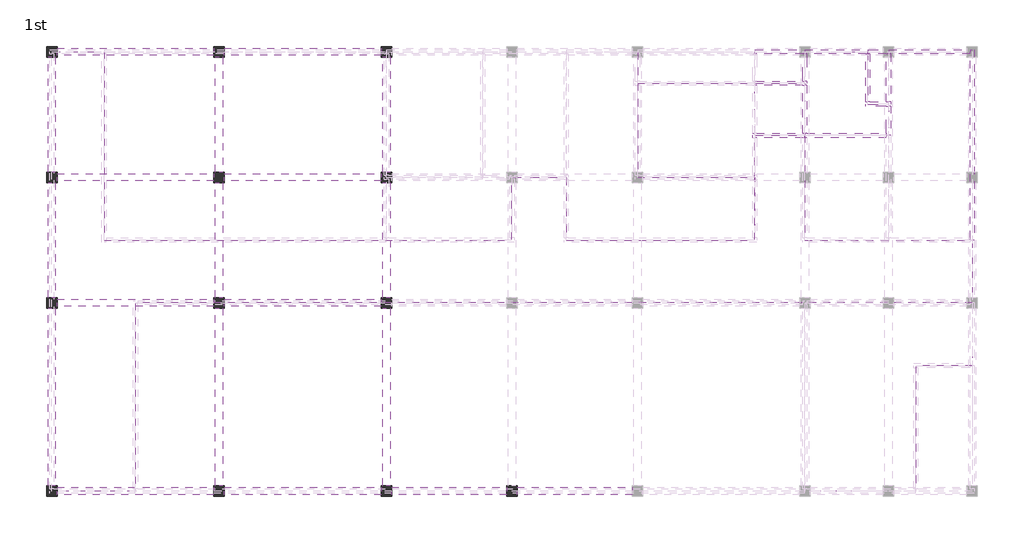
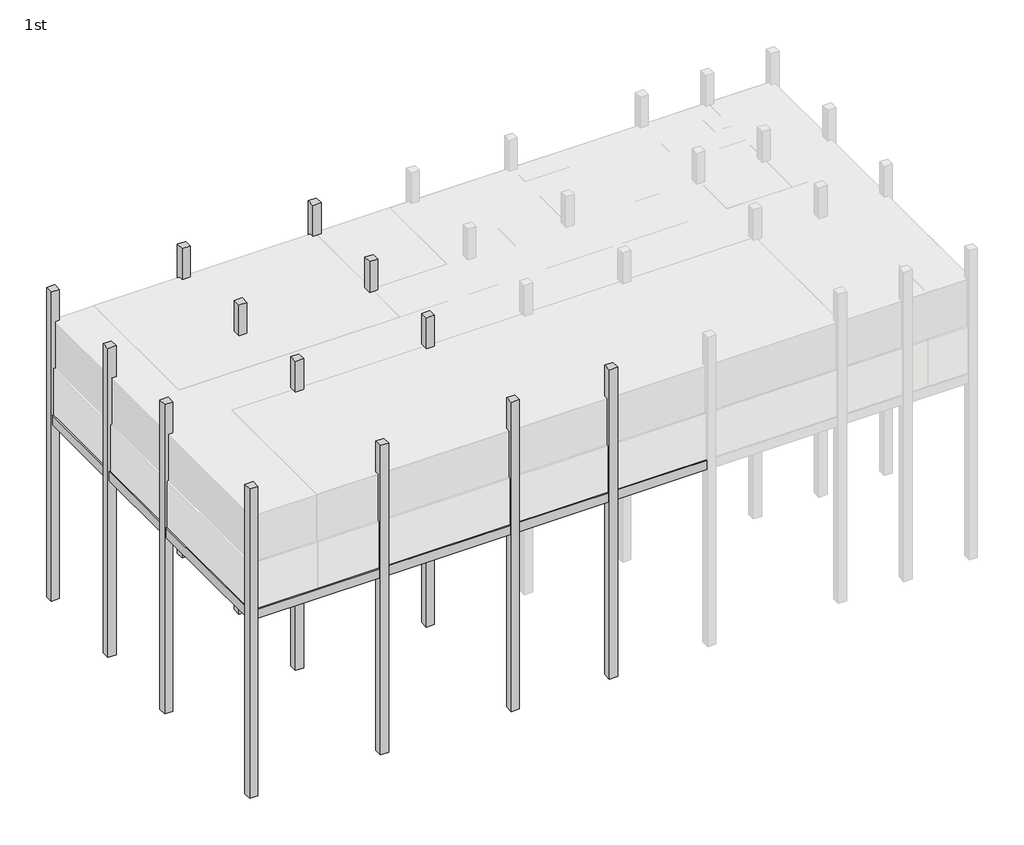
# One storey, part 2 of 3: 19 beams, 17 slabs, 14 walls, 13 columns.
"""IFC4 building model written with IfcOpenShell, lengths in millimetres."""

from ifc_helpers import new_model, si_unit, frame, origin, origin_with_axes, place, context, project, spatial, polyline, outline, extrude, faceted_brep, element, save

model = new_model("IFC4")

# Units and contexts
model_context = context("Model", 3, world=origin())
ifc_project = project(units=[si_unit("LENGTHUNIT", "METRE", prefix="MILLI")], contexts=[model_context])

# Site, building, storey
site = spatial("IfcSite", under=ifc_project)
building = spatial("IfcBuilding", under=site)
storey = spatial("IfcBuildingStorey", under=building, Name="1st", Elevation=6000.0)

# Beams
placement = place(None, origin())
element("IfcBeam", 1, ObjectType="Concrete-Rectangular-Beam : BM111_400x500_RG1", at=placement, inside=storey, context=model_context, shape_type="SweptSolid", body=[
    extrude(outline(polyline([(45284.6521483, 184673.8614395), (45634.6521483, 184673.8614395), (45634.6521483, 179173.8614395), (45284.6521483, 179173.8614395), (45284.6521483, 184673.8614395)])), frame((0.0, 0.0, 11400.0), z_axis=(0.0, 0.0, 1.0), x_axis=(1.0, 0.0, 0.0)), (0.0, 0.0, 1.0), 600.0),
])
element("IfcBeam", 2, ObjectType="Concrete-Rectangular-Beam : BM111_400x500_RG1", at=placement, inside=storey, context=model_context, shape_type="SweptSolid", body=[
    extrude(outline(polyline([(45284.6521483, 178673.8614395), (45634.6521483, 178673.8614395), (45634.6521483, 173173.8614395), (45284.6521483, 173173.8614395), (45284.6521483, 178673.8614395)])), frame((0.0, 0.0, 11400.0), z_axis=(0.0, 0.0, 1.0), x_axis=(1.0, 0.0, 0.0)), (0.0, 0.0, 1.0), 600.0),
])
element("IfcBeam", 3, ObjectType="Concrete-Rectangular-Beam : BM111_400x500_RG1", at=placement, inside=storey, context=model_context, shape_type="SweptSolid", body=[
    extrude(outline(polyline([(45284.6521483, 172673.8614395), (45634.6521483, 172673.8614395), (45634.6521483, 164173.8614395), (45284.6521483, 164173.8614395), (45284.6521483, 172673.8614395)])), frame((0.0, 0.0, 11400.0), z_axis=(0.0, 0.0, 1.0), x_axis=(1.0, 0.0, 0.0)), (0.0, 0.0, 1.0), 600.0),
])
element("IfcBeam", 4, ObjectType="Concrete-Rectangular-Beam : BM111_400x500_RG1", at=placement, inside=storey, context=model_context, shape_type="SweptSolid", body=[
    extrude(outline(polyline([(53284.6521483, 184673.8614395), (53634.6521483, 184673.8614395), (53634.6521483, 179173.8614395), (53284.6521483, 179173.8614395), (53284.6521483, 184673.8614395)])), frame((0.0, 0.0, 11400.0), z_axis=(0.0, 0.0, 1.0), x_axis=(1.0, 0.0, 0.0)), (0.0, 0.0, 1.0), 600.0),
])
element("IfcBeam", 5, ObjectType="Concrete-Rectangular-Beam : BM111_400x500_RG1", at=placement, inside=storey, context=model_context, shape_type="SweptSolid", body=[
    extrude(outline(polyline([(53284.6521483, 178673.8614395), (53634.6521483, 178673.8614395), (53634.6521483, 173173.8614395), (53284.6521483, 173173.8614395), (53284.6521483, 178673.8614395)])), frame((0.0, 0.0, 11400.0), z_axis=(0.0, 0.0, 1.0), x_axis=(1.0, 0.0, 0.0)), (0.0, 0.0, 1.0), 600.0),
])
element("IfcBeam", 6, ObjectType="Concrete-Rectangular-Beam : BM111_400x500_RG1", at=placement, inside=storey, context=model_context, shape_type="SweptSolid", body=[
    extrude(outline(polyline([(53284.6521483, 172673.8614395), (53634.6521483, 172673.8614395), (53634.6521483, 164173.8614395), (53284.6521483, 164173.8614395), (53284.6521483, 172673.8614395)])), frame((0.0, 0.0, 11400.0), z_axis=(0.0, 0.0, 1.0), x_axis=(1.0, 0.0, 0.0)), (0.0, 0.0, 1.0), 600.0),
])
element("IfcBeam", 7, ObjectType="Concrete-Rectangular-Beam : BM111_400x500_RG1", at=placement, inside=storey, context=model_context, shape_type="SweptSolid", body=[
    extrude(outline(polyline([(61284.6521483, 184673.8614395), (61634.6521483, 184673.8614395), (61634.6521483, 179173.8614395), (61284.6521483, 179173.8614395), (61284.6521483, 184673.8614395)])), frame((0.0, 0.0, 11400.0), z_axis=(0.0, 0.0, 1.0), x_axis=(1.0, 0.0, 0.0)), (0.0, 0.0, 1.0), 600.0),
])
element("IfcBeam", 8, ObjectType="Concrete-Rectangular-Beam : BM111_400x500_RG1", at=placement, inside=storey, context=model_context, shape_type="SweptSolid", body=[
    extrude(outline(polyline([(61284.6521483, 178673.8614395), (61634.6521483, 178673.8614395), (61634.6521483, 173173.8614395), (61284.6521483, 173173.8614395), (61284.6521483, 178673.8614395)])), frame((0.0, 0.0, 11400.0), z_axis=(0.0, 0.0, 1.0), x_axis=(1.0, 0.0, 0.0)), (0.0, 0.0, 1.0), 600.0),
])
element("IfcBeam", 9, ObjectType="Concrete-Rectangular-Beam : BM111_400x500_RG1", at=placement, inside=storey, context=model_context, shape_type="SweptSolid", body=[
    extrude(outline(polyline([(61284.6521483, 172673.8614395), (61634.6521483, 172673.8614395), (61634.6521483, 164173.8614395), (61284.6521483, 164173.8614395), (61284.6521483, 172673.8614395)])), frame((0.0, 0.0, 11400.0), z_axis=(0.0, 0.0, 1.0), x_axis=(1.0, 0.0, 0.0)), (0.0, 0.0, 1.0), 600.0),
])
element("IfcBeam", 10, ObjectType="Concrete-Rectangular-Beam : BM111_400x500_RG1", at=placement, inside=storey, context=model_context, shape_type="SweptSolid", body=[
    extrude(outline(polyline([(45709.6521483, 184748.8614395), (45709.6521483, 185098.8614395), (53209.6521483, 185098.8614395), (53209.6521483, 184748.8614395), (45709.6521483, 184748.8614395)])), frame((0.0, 0.0, 11400.0), z_axis=(0.0, 0.0, 1.0), x_axis=(1.0, 0.0, 0.0)), (0.0, 0.0, 1.0), 600.0),
])
element("IfcBeam", 11, ObjectType="Concrete-Rectangular-Beam : BM111_400x500_RG1", at=placement, inside=storey, context=model_context, shape_type="SweptSolid", body=[
    extrude(outline(polyline([(53709.6521483, 184748.8614395), (53709.6521483, 185098.8614395), (61209.6521483, 185098.8614395), (61209.6521483, 184748.8614395), (53709.6521483, 184748.8614395)])), frame((0.0, 0.0, 11400.0), z_axis=(0.0, 0.0, 1.0), x_axis=(1.0, 0.0, 0.0)), (0.0, 0.0, 1.0), 600.0),
])
element("IfcBeam", 12, ObjectType="Concrete-Rectangular-Beam : BM111_400x500_RG1", at=placement, inside=storey, context=model_context, shape_type="SweptSolid", body=[
    extrude(outline(polyline([(45709.6521483, 178748.8614395), (45709.6521483, 179098.8614395), (53209.6521483, 179098.8614395), (53209.6521483, 178748.8614395), (45709.6521483, 178748.8614395)])), frame((0.0, 0.0, 11400.0), z_axis=(0.0, 0.0, 1.0), x_axis=(1.0, 0.0, 0.0)), (0.0, 0.0, 1.0), 600.0),
])
element("IfcBeam", 13, ObjectType="Concrete-Rectangular-Beam : BM111_400x500_RG1", at=placement, inside=storey, context=model_context, shape_type="SweptSolid", body=[
    extrude(outline(polyline([(53709.6521483, 178748.8614395), (53709.6521483, 179098.8614395), (61209.6521483, 179098.8614395), (61209.6521483, 178748.8614395), (53709.6521483, 178748.8614395)])), frame((0.0, 0.0, 11400.0), z_axis=(0.0, 0.0, 1.0), x_axis=(1.0, 0.0, 0.0)), (0.0, 0.0, 1.0), 600.0),
])
element("IfcBeam", 14, ObjectType="Concrete-Rectangular-Beam : BM111_400x500_RG1", at=placement, inside=storey, context=model_context, shape_type="SweptSolid", body=[
    extrude(outline(polyline([(45709.6521483, 172748.8614395), (45709.6521483, 173098.8614395), (53209.6521483, 173098.8614395), (53209.6521483, 172748.8614395), (45709.6521483, 172748.8614395)])), frame((0.0, 0.0, 11400.0), z_axis=(0.0, 0.0, 1.0), x_axis=(1.0, 0.0, 0.0)), (0.0, 0.0, 1.0), 600.0),
])
element("IfcBeam", 15, ObjectType="Concrete-Rectangular-Beam : BM111_400x500_RG1", at=placement, inside=storey, context=model_context, shape_type="SweptSolid", body=[
    extrude(outline(polyline([(53709.6521483, 172748.8614395), (53709.6521483, 173098.8614395), (61209.6521483, 173098.8614395), (61209.6521483, 172748.8614395), (53709.6521483, 172748.8614395)])), frame((0.0, 0.0, 11400.0), z_axis=(0.0, 0.0, 1.0), x_axis=(1.0, 0.0, 0.0)), (0.0, 0.0, 1.0), 600.0),
])
element("IfcBeam", 16, ObjectType="Concrete-Rectangular-Beam : BM111_400x500_RG1", at=placement, inside=storey, context=model_context, shape_type="SweptSolid", body=[
    extrude(outline(polyline([(45709.6521483, 163748.8614395), (45709.6521483, 164098.8614395), (53209.6521483, 164098.8614395), (53209.6521483, 163748.8614395), (45709.6521483, 163748.8614395)])), frame((0.0, 0.0, 11400.0), z_axis=(0.0, 0.0, 1.0), x_axis=(1.0, 0.0, 0.0)), (0.0, 0.0, 1.0), 600.0),
])
element("IfcBeam", 17, ObjectType="Concrete-Rectangular-Beam : BM111_400x500_RG1", at=placement, inside=storey, context=model_context, shape_type="SweptSolid", body=[
    extrude(outline(polyline([(53709.6521483, 163748.8614395), (53709.6521483, 164098.8614395), (61209.6521483, 164098.8614395), (61209.6521483, 163748.8614395), (53709.6521483, 163748.8614395)])), frame((0.0, 0.0, 11400.0), z_axis=(0.0, 0.0, 1.0), x_axis=(1.0, 0.0, 0.0)), (0.0, 0.0, 1.0), 600.0),
])
element("IfcBeam", 18, ObjectType="Concrete-Rectangular-Beam : BM111_400x500_RG1", at=placement, inside=storey, context=model_context, shape_type="SweptSolid", body=[
    extrude(outline(polyline([(61709.6521483, 163748.8614395), (61709.6521483, 164098.8614395), (67209.6521483, 164098.8614395), (67209.6521483, 163748.8614395), (61709.6521483, 163748.8614395)])), frame((0.0, 0.0, 11400.0), z_axis=(0.0, 0.0, 1.0), x_axis=(1.0, 0.0, 0.0)), (0.0, 0.0, 1.0), 600.0),
])
element("IfcBeam", 19, ObjectType="Concrete-Rectangular-Beam : BM111_400x500_RG1", at=placement, inside=storey, context=model_context, shape_type="SweptSolid", body=[
    extrude(outline(polyline([(67709.6521483, 163748.8614395), (67709.6521483, 164098.8614395), (73209.6521483, 164098.8614395), (73209.6521483, 163748.8614395), (67709.6521483, 163748.8614395)])), frame((0.0, 0.0, 11400.0), z_axis=(0.0, 0.0, 1.0), x_axis=(1.0, 0.0, 0.0)), (0.0, 0.0, 1.0), 600.0),
])

# Columns
element("IfcColumn", 20, ObjectType="Concrete-Rectangular-Column : CL111_500x500", at=placement, inside=storey, context=model_context, shape_type="SweptSolid", body=[
    extrude(outline(polyline([(45709.6521483, 185173.8614395), (45709.6521483, 184673.8614395), (45209.6521483, 184673.8614395), (45209.6521483, 185173.8614395), (45709.6521483, 185173.8614395)])), origin_with_axes(), (0.0, 0.0, 1.0), 20000.0),
])
element("IfcColumn", 21, ObjectType="Concrete-Rectangular-Column : CL111_500x500", at=placement, inside=storey, context=model_context, shape_type="SweptSolid", body=[
    extrude(outline(polyline([(45709.6521483, 179173.8614395), (45709.6521483, 178673.8614395), (45209.6521483, 178673.8614395), (45209.6521483, 179173.8614395), (45709.6521483, 179173.8614395)])), origin_with_axes(), (0.0, 0.0, 1.0), 20000.0),
])
element("IfcColumn", 22, ObjectType="Concrete-Rectangular-Column : CL111_500x500", at=placement, inside=storey, context=model_context, shape_type="SweptSolid", body=[
    extrude(outline(polyline([(45709.6521483, 173173.8614395), (45709.6521483, 172673.8614395), (45209.6521483, 172673.8614395), (45209.6521483, 173173.8614395), (45709.6521483, 173173.8614395)])), origin_with_axes(), (0.0, 0.0, 1.0), 20000.0),
])
element("IfcColumn", 23, ObjectType="Concrete-Rectangular-Column : CL111_500x500", at=placement, inside=storey, context=model_context, shape_type="SweptSolid", body=[
    extrude(outline(polyline([(45709.6521483, 164173.8614395), (45709.6521483, 163673.8614395), (45209.6521483, 163673.8614395), (45209.6521483, 164173.8614395), (45709.6521483, 164173.8614395)])), origin_with_axes(), (0.0, 0.0, 1.0), 20000.0),
])
element("IfcColumn", 24, ObjectType="Concrete-Rectangular-Column : CL111_500x500", at=placement, inside=storey, context=model_context, shape_type="SweptSolid", body=[
    extrude(outline(polyline([(53709.6521483, 185173.8614395), (53709.6521483, 184673.8614395), (53209.6521483, 184673.8614395), (53209.6521483, 185173.8614395), (53709.6521483, 185173.8614395)])), origin_with_axes(), (0.0, 0.0, 1.0), 20000.0),
])
element("IfcColumn", 25, ObjectType="Concrete-Rectangular-Column : CL111_500x500", at=placement, inside=storey, context=model_context, shape_type="SweptSolid", body=[
    extrude(outline(polyline([(53709.6521483, 179173.8614395), (53709.6521483, 178673.8614395), (53209.6521483, 178673.8614395), (53209.6521483, 179173.8614395), (53709.6521483, 179173.8614395)])), origin_with_axes(), (0.0, 0.0, 1.0), 20000.0),
])
element("IfcColumn", 26, ObjectType="Concrete-Rectangular-Column : CL111_500x500", at=placement, inside=storey, context=model_context, shape_type="SweptSolid", body=[
    extrude(outline(polyline([(53709.6521483, 173173.8614395), (53709.6521483, 172673.8614395), (53209.6521483, 172673.8614395), (53209.6521483, 173173.8614395), (53709.6521483, 173173.8614395)])), origin_with_axes(), (0.0, 0.0, 1.0), 20000.0),
])
element("IfcColumn", 27, ObjectType="Concrete-Rectangular-Column : CL111_500x500", at=placement, inside=storey, context=model_context, shape_type="SweptSolid", body=[
    extrude(outline(polyline([(53709.6521483, 164173.8614395), (53709.6521483, 163673.8614395), (53209.6521483, 163673.8614395), (53209.6521483, 164173.8614395), (53709.6521483, 164173.8614395)])), origin_with_axes(), (0.0, 0.0, 1.0), 20000.0),
])
element("IfcColumn", 28, ObjectType="Concrete-Rectangular-Column : CL111_500x500", at=placement, inside=storey, context=model_context, shape_type="SweptSolid", body=[
    extrude(outline(polyline([(61709.6521483, 185173.8614395), (61709.6521483, 184673.8614395), (61209.6521483, 184673.8614395), (61209.6521483, 185173.8614395), (61709.6521483, 185173.8614395)])), origin_with_axes(), (0.0, 0.0, 1.0), 20000.0),
])
element("IfcColumn", 29, ObjectType="Concrete-Rectangular-Column : CL111_500x500", at=placement, inside=storey, context=model_context, shape_type="SweptSolid", body=[
    extrude(outline(polyline([(61709.6521483, 179173.8614395), (61709.6521483, 178673.8614395), (61209.6521483, 178673.8614395), (61209.6521483, 179173.8614395), (61709.6521483, 179173.8614395)])), origin_with_axes(), (0.0, 0.0, 1.0), 20000.0),
])
element("IfcColumn", 30, ObjectType="Concrete-Rectangular-Column : CL111_500x500", at=placement, inside=storey, context=model_context, shape_type="SweptSolid", body=[
    extrude(outline(polyline([(61709.6521483, 173173.8614395), (61709.6521483, 172673.8614395), (61209.6521483, 172673.8614395), (61209.6521483, 173173.8614395), (61709.6521483, 173173.8614395)])), origin_with_axes(), (0.0, 0.0, 1.0), 20000.0),
])
element("IfcColumn", 31, ObjectType="Concrete-Rectangular-Column : CL111_500x500", at=placement, inside=storey, context=model_context, shape_type="SweptSolid", body=[
    extrude(outline(polyline([(61709.6521483, 164173.8614395), (61709.6521483, 163673.8614395), (61209.6521483, 163673.8614395), (61209.6521483, 164173.8614395), (61709.6521483, 164173.8614395)])), origin_with_axes(), (0.0, 0.0, 1.0), 20000.0),
])
element("IfcColumn", 32, ObjectType="Concrete-Rectangular-Column : CL111_500x500", at=placement, inside=storey, context=model_context, shape_type="SweptSolid", body=[
    extrude(outline(polyline([(67709.6521483, 164173.8614395), (67709.6521483, 163673.8614395), (67209.6521483, 163673.8614395), (67209.6521483, 164173.8614395), (67709.6521483, 164173.8614395)])), origin_with_axes(), (0.0, 0.0, 1.0), 20000.0),
])

# Slabs
element("IfcSlab", 33, ObjectType="CFS11_Slab RC_T150", at=placement, inside=storey, context=model_context, shape_type="SweptSolid", body=[
    extrude(outline(polyline([(49459.6521483, 172923.8614395), (81459.6521483, 172923.8614395), (81459.6521483, 163923.8614395), (49459.6521483, 163923.8614395), (49459.6521483, 172923.8614395)])), frame((0.0, 0.0, 11850.0), z_axis=(0.0, 0.0, 1.0), x_axis=(1.0, 0.0, 0.0)), (0.0, 0.0, 1.0), 150.0),
])
element("IfcSlab", 34, ObjectType="CFS11_Slab RC_T150", at=placement, inside=storey, context=model_context, shape_type="SweptSolid", body=[
    extrude(outline(polyline([(47959.6521483, 184923.8614395), (61459.6521483, 184923.8614395), (61459.6521483, 175923.8614395), (47959.6521483, 175923.8614395), (47959.6521483, 184923.8614395)])), frame((0.0, 0.0, 11850.0), z_axis=(0.0, 0.0, 1.0), x_axis=(1.0, 0.0, 0.0)), (0.0, 0.0, 1.0), 150.0),
])
element("IfcSlab", 35, ObjectType="CFS11_Slab RC_T150", at=placement, inside=storey, context=model_context, shape_type="SweptSolid", body=[
    extrude(outline(polyline([(61459.6521483, 178923.8614395), (61459.6521483, 184923.8614395), (66059.6521483, 184923.8614395), (66059.6521483, 178923.8614395), (61459.6521483, 178923.8614395)])), frame((0.0, 0.0, 11850.0), z_axis=(0.0, 0.0, 1.0), x_axis=(1.0, 0.0, 0.0)), (0.0, 0.0, 1.0), 150.0),
])
element("IfcSlab", 36, ObjectType="CFS11_Slab RC_T150", at=placement, inside=storey, context=model_context, shape_type="SweptSolid", body=[
    extrude(outline(polyline([(81459.6521483, 175923.8614395), (81459.6521483, 180923.8614395), (85459.6521483, 180923.8614395), (85459.6521483, 175923.8614395), (81459.6521483, 175923.8614395)])), frame((0.0, 0.0, 11850.0), z_axis=(0.0, 0.0, 1.0), x_axis=(1.0, 0.0, 0.0)), (0.0, 0.0, 1.0), 150.0),
])
element("IfcSlab", 37, ObjectType="CFS11_Slab RC_T150", at=placement, inside=storey, context=model_context, shape_type="SweptSolid", body=[
    extrude(outline(polyline([(89459.6521483, 175923.8614395), (85459.6521483, 175923.8614395), (85459.6521483, 184923.8614395), (89459.6521483, 184923.8614395), (89459.6521483, 175923.8614395)])), frame((0.0, 0.0, 11850.0), z_axis=(0.0, 0.0, 1.0), x_axis=(1.0, 0.0, 0.0)), (0.0, 0.0, 1.0), 150.0),
])
element("IfcSlab", 38, ObjectType="CFS11_Slab RC_T150", at=placement, inside=storey, context=model_context, shape_type="SweptSolid", body=[
    extrude(outline(polyline([(66059.6521483, 178923.8614395), (66059.6521483, 184923.8614395), (70059.6521483, 184923.8614395), (70059.6521483, 178923.8614395), (66059.6521483, 178923.8614395)])), frame((0.0, 0.0, 11850.0), z_axis=(0.0, 0.0, 1.0), x_axis=(1.0, 0.0, 0.0)), (0.0, 0.0, 1.0), 150.0),
])
element("IfcSlab", 39, ObjectType="CFS11_Slab RC_T150", at=placement, inside=storey, context=model_context, shape_type="SweptSolid", body=[
    extrude(outline(polyline([(61459.6521483, 175923.8614395), (61459.6521483, 178923.8614395), (67459.6521483, 178923.8614395), (67459.6521483, 175923.8614395), (61459.6521483, 175923.8614395)])), frame((0.0, 0.0, 11850.0), z_axis=(0.0, 0.0, 1.0), x_axis=(1.0, 0.0, 0.0)), (0.0, 0.0, 1.0), 150.0),
])
element("IfcSlab", 40, ObjectType="CFS11_Slab RC_T150", at=placement, inside=storey, context=model_context, shape_type="SweptSolid", body=[
    extrude(outline(polyline([(79059.6521483, 183423.8614395), (79059.6521483, 184923.8614395), (81459.6521483, 184923.8614395), (81459.6521483, 183423.8614395), (79059.6521483, 183423.8614395)])), frame((0.0, 0.0, 11850.0), z_axis=(0.0, 0.0, 1.0), x_axis=(1.0, 0.0, 0.0)), (0.0, 0.0, 1.0), 150.0),
])
element("IfcSlab", 41, ObjectType="CFS11_Slab RC_T150", at=placement, inside=storey, context=model_context, shape_type="SweptSolid", body=[
    extrude(outline(polyline([(89459.6521483, 172923.8614395), (49459.6521483, 172923.8614395), (49459.6521483, 163923.8614395), (45459.6521483, 163923.8614395), (45459.6521483, 184923.8614395), (47959.6521483, 184923.8614395), (47959.6521483, 175923.8614395), (67459.6521483, 175923.8614395), (67459.6521483, 178923.8614395), (70059.6521483, 178923.8614395), (70059.6521483, 175923.8614395), (79059.6521483, 175923.8614395), (79059.6521483, 180923.8614395), (81459.6521483, 180923.8614395), (81459.6521483, 175923.8614395), (89459.6521483, 175923.8614395), (89459.6521483, 172923.8614395)])), frame((0.0, 0.0, 11850.0), z_axis=(0.0, 0.0, 1.0), x_axis=(1.0, 0.0, 0.0)), (0.0, 0.0, 1.0), 150.0),
])
element("IfcSlab", 42, ObjectType="CFS11_Slab RC_T150", at=placement, inside=storey, context=model_context, shape_type="SweptSolid", body=[
    extrude(outline(polyline([(79059.6521483, 180923.8614395), (79059.6521483, 183423.8614395), (81459.6521483, 183423.8614395), (81459.6521483, 180923.8614395), (79059.6521483, 180923.8614395)])), frame((0.0, 0.0, 11850.0), z_axis=(0.0, 0.0, 1.0), x_axis=(1.0, 0.0, 0.0)), (0.0, 0.0, 1.0), 150.0),
])
element("IfcSlab", 43, ObjectType="CFS11_Slab RC_T150", at=placement, inside=storey, context=model_context, shape_type="SweptSolid", body=[
    extrude(outline(polyline([(73459.6521483, 184923.8614395), (79059.6521483, 184923.8614395), (79059.6521483, 183423.8614395), (73459.6521483, 183423.8614395), (73459.6521483, 184923.8614395)])), frame((0.0, 0.0, 11850.0), z_axis=(0.0, 0.0, 1.0), x_axis=(1.0, 0.0, 0.0)), (0.0, 0.0, 1.0), 150.0),
])
element("IfcSlab", 44, ObjectType="CFS11_Slab RC_T150", at=placement, inside=storey, context=model_context, shape_type="SweptSolid", body=[
    extrude(outline(polyline([(79059.6521483, 175923.8614395), (70059.6521483, 175923.8614395), (70059.6521483, 184923.8614395), (73459.6521483, 184923.8614395), (73459.6521483, 178923.8614395), (79059.6521483, 178923.8614395), (79059.6521483, 175923.8614395)])), frame((0.0, 0.0, 11850.0), z_axis=(0.0, 0.0, 1.0), x_axis=(1.0, 0.0, 0.0)), (0.0, 0.0, 1.0), 150.0),
])
element("IfcSlab", 45, ObjectType="CFS11_Slab RC_T150", at=placement, inside=storey, context=model_context, shape_type="SweptSolid", body=[
    extrude(outline(polyline([(73459.6521483, 183423.8614395), (79059.6521483, 183423.8614395), (79059.6521483, 178923.8614395), (73459.6521483, 178923.8614395), (73459.6521483, 183423.8614395)])), frame((0.0, 0.0, 11850.0), z_axis=(0.0, 0.0, 1.0), x_axis=(1.0, 0.0, 0.0)), (0.0, 0.0, 1.0), 150.0),
])
element("IfcSlab", 46, ObjectType="CFS11_Slab RC_T150", at=placement, inside=storey, context=model_context, shape_type="SweptSolid", body=[
    extrude(outline(polyline([(81459.6521483, 163923.8614395), (81459.6521483, 172923.8614395), (89459.6521483, 172923.8614395), (89459.6521483, 169923.8614395), (86759.6521483, 169923.8614395), (86759.6521483, 163923.8614395), (81459.6521483, 163923.8614395)])), frame((0.0, 0.0, 11850.0), z_axis=(0.0, 0.0, 1.0), x_axis=(1.0, 0.0, 0.0)), (0.0, 0.0, 1.0), 150.0),
])
element("IfcSlab", 47, ObjectType="CFS11_Slab RC_T150", at=placement, inside=storey, context=model_context, shape_type="SweptSolid", body=[
    extrude(outline(polyline([(89459.6521483, 169923.8614395), (89459.6521483, 163923.8614395), (86759.6521483, 163923.8614395), (86759.6521483, 169923.8614395), (89459.6521483, 169923.8614395)])), frame((0.0, 0.0, 11850.0), z_axis=(0.0, 0.0, 1.0), x_axis=(1.0, 0.0, 0.0)), (0.0, 0.0, 1.0), 150.0),
])
element("IfcSlab", 48, ObjectType="CFS11_Slab RC_T150", at=placement, inside=storey, context=model_context, shape_type="SweptSolid", body=[
    extrude(outline(polyline([(85459.6521483, 180923.8614395), (81459.6521483, 180923.8614395), (81459.6521483, 184923.8614395), (84459.6521483, 184923.8614395), (84459.6521483, 182423.8614395), (85459.6521483, 182423.8614395), (85459.6521483, 180923.8614395)])), frame((0.0, 0.0, 11850.0), z_axis=(0.0, 0.0, 1.0), x_axis=(1.0, 0.0, 0.0)), (0.0, 0.0, 1.0), 150.0),
])
element("IfcSlab", 49, ObjectType="CFS11_Slab RC_T150", at=placement, inside=storey, context=model_context, shape_type="SweptSolid", body=[
    extrude(outline(polyline([(84459.6521483, 184923.8614395), (85459.6521483, 184923.8614395), (85459.6521483, 182423.8614395), (84459.6521483, 182423.8614395), (84459.6521483, 184923.8614395)])), frame((0.0, 0.0, 11850.0), z_axis=(0.0, 0.0, 1.0), x_axis=(1.0, 0.0, 0.0)), (0.0, 0.0, 1.0), 150.0),
])

# Walls
element("IfcWall", 50, ObjectType="WA111-Exterior RC Wall 200mm", at=placement, inside=storey, context=model_context, shape_type="Brep", body=[
    faceted_brep([(89559.6521483, 175923.8614395, 12000.0), (89559.6521483, 185023.8614395, 12000.0), (89559.6521483, 185023.8614395, 15000.0), (89559.6521483, 175923.8614395, 15000.0), (89359.6521483, 175923.8614395, 12000.0), (89359.6521483, 175923.8614395, 15000.0), (89359.6521483, 176023.8614395, 15000.0), (89359.6521483, 184823.8614395, 15000.0), (89359.6521483, 185023.8614395, 15000.0), (89359.6521483, 185023.8614395, 12000.0), (89359.6521483, 184823.8614395, 12000.0), (89359.6521483, 176023.8614395, 12000.0)], [[[0, 1, 2, 3]], [[4, 5, 6, 7, 8, 9, 10, 11]], [[1, 0, 4, 11, 10, 9]], [[3, 2, 8, 7, 6, 5]], [[0, 3, 5, 4]], [[2, 1, 9, 8]]]),
])
element("IfcWall", 51, ObjectType="WA111-Exterior RC Wall 200mm", at=placement, inside=storey, context=model_context, shape_type="Brep", body=[
    faceted_brep([(89359.6521483, 185023.8614395, 12000.0), (85459.6521483, 185023.8614395, 12000.0), (85459.6521483, 185023.8614395, 15000.0), (89359.6521483, 185023.8614395, 15000.0), (89359.6521483, 184823.8614395, 12000.0), (89359.6521483, 184823.8614395, 15000.0), (85559.6521483, 184823.8614395, 15000.0), (85459.6521483, 184823.8614395, 15000.0), (85459.6521483, 184823.8614395, 12000.0), (85559.6521483, 184823.8614395, 12000.0)], [[[0, 1, 2, 3]], [[4, 5, 6, 7, 8, 9]], [[1, 0, 4, 9, 8]], [[2, 1, 8, 7]], [[3, 2, 7, 6, 5]], [[0, 3, 5, 4]]]),
])
element("IfcWall", 52, ObjectType="WA111-Exterior RC Wall 200mm", at=placement, inside=storey, context=model_context, shape_type="Brep", body=[
    faceted_brep([(81459.6521483, 185023.8614395, 12000.0), (79059.6521483, 185023.8614395, 12000.0), (79059.6521483, 185023.8614395, 15000.0), (81459.6521483, 185023.8614395, 15000.0), (81459.6521483, 184823.8614395, 12000.0), (81459.6521483, 184823.8614395, 15000.0), (81359.6521483, 184823.8614395, 15000.0), (79159.6521483, 184823.8614395, 15000.0), (79059.6521483, 184823.8614395, 15000.0), (79059.6521483, 184823.8614395, 12000.0), (79159.6521483, 184823.8614395, 12000.0), (81359.6521483, 184823.8614395, 12000.0)], [[[0, 1, 2, 3]], [[4, 5, 6, 7, 8, 9, 10, 11]], [[1, 0, 4, 11, 10, 9]], [[2, 1, 9, 8]], [[3, 2, 8, 7, 6, 5]], [[0, 3, 5, 4]]]),
])
element("IfcWall", 53, ObjectType="WA111-Exterior RC Wall 200mm", at=placement, inside=storey, context=model_context, shape_type="Brep", body=[
    faceted_brep([(84459.6521483, 185023.8614395, 12000.0), (81459.6521483, 185023.8614395, 12000.0), (81459.6521483, 185023.8614395, 15000.0), (84459.6521483, 185023.8614395, 15000.0), (84459.6521483, 184823.8614395, 12000.0), (84459.6521483, 184823.8614395, 15000.0), (84359.6521483, 184823.8614395, 15000.0), (81559.6521483, 184823.8614395, 15000.0), (81459.6521483, 184823.8614395, 15000.0), (81459.6521483, 184823.8614395, 12000.0), (81559.6521483, 184823.8614395, 12000.0), (84359.6521483, 184823.8614395, 12000.0)], [[[0, 1, 2, 3]], [[4, 5, 6, 7, 8, 9, 10, 11]], [[1, 0, 4, 11, 10, 9]], [[2, 1, 9, 8]], [[3, 2, 8, 7, 6, 5]], [[0, 3, 5, 4]]]),
])
element("IfcWall", 54, ObjectType="WA111-Exterior RC Wall 200mm", at=placement, inside=storey, context=model_context, shape_type="Brep", body=[
    faceted_brep([(85459.6521483, 185023.8614395, 12000.0), (84459.6521483, 185023.8614395, 12000.0), (84459.6521483, 185023.8614395, 15000.0), (85459.6521483, 185023.8614395, 15000.0), (85459.6521483, 184823.8614395, 12000.0), (85459.6521483, 184823.8614395, 15000.0), (85359.6521483, 184823.8614395, 15000.0), (84559.6521483, 184823.8614395, 15000.0), (84459.6521483, 184823.8614395, 15000.0), (84459.6521483, 184823.8614395, 12000.0), (84559.6521483, 184823.8614395, 12000.0), (85359.6521483, 184823.8614395, 12000.0)], [[[0, 1, 2, 3]], [[4, 5, 6, 7, 8, 9, 10, 11]], [[1, 0, 4, 11, 10, 9]], [[2, 1, 9, 8]], [[3, 2, 8, 7, 6, 5]], [[0, 3, 5, 4]]]),
])
element("IfcWall", 55, ObjectType="WA121-Interior RC Wall 200mm", at=placement, inside=storey, context=model_context, shape_type="Brep", body=[
    faceted_brep([(85359.6521483, 181023.8614395, 12000.0), (81559.6521483, 181023.8614395, 12000.0), (81459.6521483, 181023.8614395, 12000.0), (81459.6521483, 181023.8614395, 15000.0), (81559.6521483, 181023.8614395, 15000.0), (85359.6521483, 181023.8614395, 15000.0), (85359.6521483, 180823.8614395, 12000.0), (85359.6521483, 180823.8614395, 15000.0), (81559.6521483, 180823.8614395, 15000.0), (81459.6521483, 180823.8614395, 15000.0), (81459.6521483, 180823.8614395, 12000.0), (81559.6521483, 180823.8614395, 12000.0), (85359.6521483, 180923.8614395, 12000.0), (85359.6521483, 180923.8614395, 15000.0)], [[[0, 1, 2, 3, 4, 5]], [[6, 7, 8, 9, 10, 11]], [[2, 1, 0, 12, 6, 11, 10]], [[3, 2, 10, 9]], [[5, 4, 3, 9, 8, 7, 13]], [[0, 5, 13, 7, 6, 12]]]),
])
element("IfcWall", 56, ObjectType="WA121-Interior RC Wall 200mm", at=placement, inside=storey, context=model_context, shape_type="Brep", body=[
    faceted_brep([(85359.6521483, 184823.8614395, 12000.0), (85359.6521483, 182523.8614395, 12000.0), (85359.6521483, 182523.8614395, 15000.0), (85359.6521483, 184823.8614395, 15000.0), (85559.6521483, 184823.8614395, 12000.0), (85559.6521483, 184823.8614395, 15000.0), (85559.6521483, 182523.8614395, 15000.0), (85559.6521483, 182523.8614395, 12000.0), (85459.6521483, 184823.8614395, 12000.0), (85459.6521483, 184823.8614395, 15000.0)], [[[0, 1, 2, 3]], [[4, 5, 6, 7]], [[1, 0, 8, 4, 7]], [[3, 2, 6, 5, 9]], [[0, 3, 9, 5, 4, 8]], [[2, 1, 7, 6]]]),
])
element("IfcWall", 57, ObjectType="WA121-Interior RC Wall 200mm", at=placement, inside=storey, context=model_context, shape_type="Brep", body=[
    faceted_brep([(85359.6521483, 182323.8614395, 12000.0), (85359.6521483, 181023.8614395, 12000.0), (85359.6521483, 180923.8614395, 12000.0), (85359.6521483, 180923.8614395, 15000.0), (85359.6521483, 181023.8614395, 15000.0), (85359.6521483, 182323.8614395, 15000.0), (85559.6521483, 182323.8614395, 12000.0), (85559.6521483, 182323.8614395, 15000.0), (85559.6521483, 180923.8614395, 15000.0), (85559.6521483, 180923.8614395, 12000.0)], [[[0, 1, 2, 3, 4, 5]], [[6, 7, 8, 9]], [[2, 1, 0, 6, 9]], [[3, 2, 9, 8]], [[5, 4, 3, 8, 7]], [[0, 5, 7, 6]]]),
])
element("IfcWall", 58, ObjectType="WA121-Interior RC Wall 200mm", at=placement, inside=storey, context=model_context, shape_type="Brep", body=[
    faceted_brep([(79059.6521483, 183323.8614395, 12000.0), (79159.6521483, 183323.8614395, 12000.0), (81359.6521483, 183323.8614395, 12000.0), (81559.6521483, 183323.8614395, 12000.0), (81559.6521483, 183323.8614395, 15000.0), (81359.6521483, 183323.8614395, 15000.0), (79159.6521483, 183323.8614395, 15000.0), (79059.6521483, 183323.8614395, 15000.0), (79059.6521483, 183523.8614395, 12000.0), (79059.6521483, 183523.8614395, 15000.0), (79159.6521483, 183523.8614395, 15000.0), (81359.6521483, 183523.8614395, 15000.0), (81559.6521483, 183523.8614395, 15000.0), (81559.6521483, 183523.8614395, 12000.0), (81359.6521483, 183523.8614395, 12000.0), (79159.6521483, 183523.8614395, 12000.0)], [[[0, 1, 2, 3, 4, 5, 6, 7]], [[8, 9, 10, 11, 12, 13, 14, 15]], [[3, 2, 1, 0, 8, 15, 14, 13]], [[7, 6, 5, 4, 12, 11, 10, 9]], [[0, 7, 9, 8]], [[4, 3, 13, 12]]]),
])
element("IfcWall", 59, ObjectType="WA121-Interior RC Wall 200mm", at=placement, inside=storey, context=model_context, shape_type="Brep", body=[
    faceted_brep([(81559.6521483, 183523.8614395, 12000.0), (81559.6521483, 184823.8614395, 12000.0), (81559.6521483, 184823.8614395, 15000.0), (81559.6521483, 183523.8614395, 15000.0), (81359.6521483, 183523.8614395, 12000.0), (81359.6521483, 183523.8614395, 15000.0), (81359.6521483, 184823.8614395, 15000.0), (81359.6521483, 184823.8614395, 12000.0), (81459.6521483, 184823.8614395, 12000.0), (81459.6521483, 184823.8614395, 15000.0)], [[[0, 1, 2, 3]], [[4, 5, 6, 7]], [[1, 0, 4, 7, 8]], [[3, 2, 9, 6, 5]], [[2, 1, 8, 7, 6, 9]], [[0, 3, 5, 4]]]),
])
element("IfcWall", 60, ObjectType="WA121-Interior RC Wall 200mm", at=placement, inside=storey, context=model_context, shape_type="Brep", body=[
    faceted_brep([(81459.6521483, 181023.8614395, 12000.0), (81359.6521483, 181023.8614395, 12000.0), (79159.6521483, 181023.8614395, 12000.0), (78959.6521483, 181023.8614395, 12000.0), (78959.6521483, 181023.8614395, 15000.0), (79159.6521483, 181023.8614395, 15000.0), (81359.6521483, 181023.8614395, 15000.0), (81459.6521483, 181023.8614395, 15000.0), (81459.6521483, 180823.8614395, 12000.0), (81459.6521483, 180823.8614395, 15000.0), (81359.6521483, 180823.8614395, 15000.0), (79159.6521483, 180823.8614395, 15000.0), (78959.6521483, 180823.8614395, 15000.0), (78959.6521483, 180823.8614395, 12000.0), (79159.6521483, 180823.8614395, 12000.0), (81359.6521483, 180823.8614395, 12000.0)], [[[0, 1, 2, 3, 4, 5, 6, 7]], [[8, 9, 10, 11, 12, 13, 14, 15]], [[3, 2, 1, 0, 8, 15, 14, 13]], [[7, 6, 5, 4, 12, 11, 10, 9]], [[0, 7, 9, 8]], [[4, 3, 13, 12]]]),
])
element("IfcWall", 61, ObjectType="WA121-Interior RC Wall 200mm", at=placement, inside=storey, context=model_context, shape_type="Brep", body=[
    faceted_brep([(81559.6521483, 181023.8614395, 12000.0), (81559.6521483, 183323.8614395, 12000.0), (81559.6521483, 183323.8614395, 15000.0), (81559.6521483, 181023.8614395, 15000.0), (81359.6521483, 181023.8614395, 12000.0), (81359.6521483, 181023.8614395, 15000.0), (81359.6521483, 183323.8614395, 15000.0), (81359.6521483, 183323.8614395, 12000.0), (81459.6521483, 181023.8614395, 12000.0), (81459.6521483, 181023.8614395, 15000.0)], [[[0, 1, 2, 3]], [[4, 5, 6, 7]], [[1, 0, 8, 4, 7]], [[3, 2, 6, 5, 9]], [[0, 3, 9, 5, 4, 8]], [[2, 1, 7, 6]]]),
])
element("IfcWall", 62, ObjectType="WA121-Interior RC Wall 200mm", at=placement, inside=storey, context=model_context, shape_type="Brep", body=[
    faceted_brep([(85559.6521483, 182523.8614395, 12000.0), (85359.6521483, 182523.8614395, 12000.0), (84559.6521483, 182523.8614395, 12000.0), (84359.6521483, 182523.8614395, 12000.0), (84359.6521483, 182523.8614395, 15000.0), (84559.6521483, 182523.8614395, 15000.0), (85359.6521483, 182523.8614395, 15000.0), (85559.6521483, 182523.8614395, 15000.0), (85559.6521483, 182323.8614395, 12000.0), (85559.6521483, 182323.8614395, 15000.0), (85359.6521483, 182323.8614395, 15000.0), (84359.6521483, 182323.8614395, 15000.0), (84359.6521483, 182323.8614395, 12000.0), (85359.6521483, 182323.8614395, 12000.0)], [[[0, 1, 2, 3, 4, 5, 6, 7]], [[8, 9, 10, 11, 12, 13]], [[3, 2, 1, 0, 8, 13, 12]], [[7, 6, 5, 4, 11, 10, 9]], [[4, 3, 12, 11]], [[0, 7, 9, 8]]]),
])
element("IfcWall", 63, ObjectType="WA121-Interior RC Wall 200mm", at=placement, inside=storey, context=model_context, shape_type="Brep", body=[
    faceted_brep([(84559.6521483, 182523.8614395, 12000.0), (84559.6521483, 184823.8614395, 12000.0), (84559.6521483, 184823.8614395, 15000.0), (84559.6521483, 182523.8614395, 15000.0), (84359.6521483, 182523.8614395, 12000.0), (84359.6521483, 182523.8614395, 15000.0), (84359.6521483, 184823.8614395, 15000.0), (84359.6521483, 184823.8614395, 12000.0), (84459.6521483, 184823.8614395, 12000.0), (84459.6521483, 184823.8614395, 15000.0)], [[[0, 1, 2, 3]], [[4, 5, 6, 7]], [[1, 0, 4, 7, 8]], [[3, 2, 9, 6, 5]], [[2, 1, 8, 7, 6, 9]], [[0, 3, 5, 4]]]),
])

save(model, "model.ifc")

# Revit data of these elements
# Type "Concrete-Rectangular-Beam : BM111_400x500_RG1"
#   중앙부 하부근 = "3-D20"
#   중앙부 상부근 = "3-D20"
#   중앙부 보조근 = ""
#   중앙부 늑근 = "2-D10 @200"
#   외단부 하부근 = "3-D20"
#   외단부 상부근 = "3-D20"
#   외단부 보조근 = ""
#   외단부 늑근 = "2-D10 @100"
#   부호 = "RG1"
#   내단부 하부근 = "3-D20"
#   내단부 상부근 = "3-D20"
#   내단부 보조근 = ""
#   내단부 늑근 = "2-D10 @100"
#   ALL 하부근 = ""
#   ALL 상부근 = ""
#   ALL 보조근 = ""
#   ALL 늑근 = ""
#   Width = 400 mm
#   Height = 500 mm
#   Length [instance default] = 1524 mm
#   Structural Material [instance default] = 콘크리트 - 현장타설 콘크리트
#   hec_material3 [instance default] = none
#   hec_material2 [instance default] = none
#   hec_material1 [instance default] = none
#   Assembly Code = ""
# Type "Concrete-Rectangular-Column : CL111_500x500"
#   Description = "UG 철골 기둥용 Pedestal"
#   b = 500 mm
#   h = 500 mm
#   hec_material3 [instance default] = none
#   hec_material2 [instance default] = A03AE056-00001_Bitumen/Bituminous/Asphalt Coating
#   hec_material1 [instance default] = A03AC035-00001_Form Work (3 times in use)_Flat
#   Structural Material [instance default] = A03AC032-00007_Structural Concrete_Type1_25MPa-30Mpa
# Type "CFS11_Slab RC_T150"
#   Keynote = ""
#   Type Comments = "구조_콘크리트"
#   Function = 0
#   Layers, outside or top first: 150 mm "14200-030101_Concrete Pouring" (function 1)
# Type "WA111-Exterior RC Wall 200mm"
#   Type Comments = ""
#   Layers, outside or top first: 0 mm "A04AL077-00001_Ext Wall Painting_Acrylic Emulsion Paint" (function 100); 200 mm "A03AD032-00007_Structural Concrete_25MPa-30MPa" (function 1); 0 mm "A03AD036-00001_Form Work (1 time in use)" (function 100); 0 mm "A04AL078-00002_Int Wall Painting_Water Emulsion Paint" (function 100); 0 mm "A04AL081-00001_Skirt_Acrylic Emulsion Paint" (function 100)
# Type "WA121-Interior RC Wall 200mm"
#   Type Comments = ""
#   Layers, outside or top first: 0 mm "A04AL081-00001_Skirt_Acrylic Emulsion Paint" (function 100); 0 mm "A04AL078-00002_Int Wall Painting_Water Emulsion Paint" (function 100); 200 mm "A03AD032-00007_Structural Concrete_25MPa-30MPa" (function 1); 0 mm "A03AD036-00001_Form Work (1 time in use)" (function 100); 0 mm "A04AL078-00002_Int Wall Painting_Water Emulsion Paint" (function 100); 0 mm "A04AL081-00001_Skirt_Acrylic Emulsion Paint" (function 100)
# Elements 1, 2, 3, 4, 5, 6, 7, 8, 9, 10, 11, 12, 13, 14, 15, 16, 17, 18, 19 (IfcBeam, "Concrete-Rectangular-Beam : BM111_400x500_RG1")
#   Comments = ""
#   hec_material3 = none
#   hec_material2 = none
#   hec_material1 = none
#   Structural Material = 콘크리트 - 현장타설 콘크리트
#   Phase Created = New Construction
#   Materials on its faces: "콘크리트 - 현장타설 콘크리트"
# Elements 20, 21, 22, 23, 24, 25, 26, 27, 28, 29, 30, 31, 32 (IfcColumn, "Concrete-Rectangular-Column : CL111_500x500")
#   Comments = ""
#   hec_material3 = none
#   hec_material2 = none
#   hec_material1 = none
#   Structural Material = 콘크리트 - 현장타설 콘크리트
#   Phase Created = New Construction
#   Materials on its faces: "콘크리트 - 현장타설 콘크리트"
# Elements 33, 34, 35, 36, 37, 38, 39, 40, 41, 42, 43, 44, 45, 46, 47, 48, 49 (IfcSlab, "CFS11_Slab RC_T150")
#   Height Offset From Level = 0 mm
#   Phase Created = New Construction
#   Materials on its faces: "14200-030101_Concrete Pouring"
# Element 50 (IfcWall, "WA111-Exterior RC Wall 200mm")
#   Top Offset = -1200 mm
#   Base Offset = 0 mm
#   Unconnected Height = 3000 mm
#   wall height = 3000 mm
#   Phase Created = New Construction
#   Base Constraint = 2nd
#   Materials on its faces: "A03AD032-00007_Structural Concrete_25MPa-30MPa", "Default Wall"
# Elements 51, 52, 53, 54 (IfcWall, "WA111-Exterior RC Wall 200mm")
#   Top Offset = -1200 mm
#   Base Offset = 0 mm
#   Unconnected Height = 3000 mm
#   wall height = 3000 mm
#   Phase Created = New Construction
#   Base Constraint = 2nd
#   Materials on its faces: "Default Wall", "A03AD032-00007_Structural Concrete_25MPa-30MPa"
# Elements 55, 56, 57, 59, 61, 63 (IfcWall, "WA121-Interior RC Wall 200mm")
#   Top Offset = 0 mm
#   Base Offset = 0 mm
#   Unconnected Height = 3000 mm
#   wall height = 3000 mm
#   Phase Created = New Construction
#   Base Constraint = 2nd
#   Materials on its faces: "Default Wall", "A03AD032-00007_Structural Concrete_25MPa-30MPa"
# Elements 58, 60, 62 (IfcWall, "WA121-Interior RC Wall 200mm")
#   Top Offset = 0 mm
#   Base Offset = 0 mm
#   Unconnected Height = 3000 mm
#   wall height = 3000 mm
#   Phase Created = New Construction
#   Base Constraint = 2nd
#   Materials on its faces: "A03AD032-00007_Structural Concrete_25MPa-30MPa", "Default Wall"
# Materials
#   "콘크리트 - 현장타설 콘크리트": class "콘크리트", colour RGB 192 192 192, transparency 0
#   "A03AE056-00001_Bitumen/Bituminous/Asphalt Coating": class "Generic", colour RGB 17 17 17, transparency 0, Description = "Damp-proofing", W00) Work Master Code = "A03AE056-00001", W01) Work Master_Lv1 = "Concrete Work", W02) Work Master_Lv2 = "Concrete Protective Coating (U/G)", W03) Work Master_Spec.1 = "Bitumen/Bituminous/Asphalt Coating", Cost = 0
#   "A03AC035-00001_Form Work (3 times in use)_Flat": class "Wood", colour RGB 149 120 74, transparency 0, Description = "Plywood", W00) Work Master Code = "A03AC035-00001", W01) Work Master_Lv1 = "Concrete Work", W02) Work Master_Lv2 = "Substructure Work", W03) Work Master_Spec.1 = "Form Work (3 times in use)", W04) Work Master_Spec.2 = "Flat Form", W05) Work Master_Spec.3 = "Dressed Lumber, Plywood or Steel Form(Wood Planks are not Allowed) incl. Chamfer", Cost = 0
#   "A03AC032-00007_Structural Concrete_Type1_25MPa-30Mpa": class "Concrete", colour RGB 176 176 176, transparency 0, Keynote = "09910.A1", Description = "Reinf. Conc.", W00) Work Master Code = "A03AC032-00007", W01) Work Master_Lv1 = "Concrete Work", W02) Work Master_Lv2 = "Substructure Work", W03) Work Master_Spec.1 = "Structural Concrete", W04) Work Master_Spec.2 = "Cement Type-1", W05) Work Master_Spec.3 = "25MPa < F'c (Cylinder Strength) ≤ 30MPa", Cost = 0
#   "14200-030101_Concrete Pouring": class "Concrete", colour RGB 176 176 176, transparency 0, Description = "Reinf. Conc.", W00) Work Master Code = "14200-030101", W01) Work Master_Lv1 = "Concrete Work", W02) Work Master_Lv2 = "Building/Shelter Foundation Work", W03) Work Master_Spec.1 = "Concrete Pouring", W04) Work Master_Spec.2 = "F'c (Cylinder Strength) > 35MPa", W05) Work Master_Spec.3 = "Cement Type-1", Cost = 0
#   "A04AL077-00001_Ext Wall Painting_Acrylic Emulsion Paint": class "Finish", colour RGB 128 128 64, transparency 0, Description = "Plastic", W00) Work Master Code = "A04AL077-00001", W01) Work Master_Lv1 = "Finishing Work", W02) Work Master_Lv2 = "Painting Work", W03) Work Master_Spec.1 = "External Wall Painting", W04) Work Master_Spec.2 = "Acrylic Emulsion Paint", Cost = 0
#   "A03AD032-00007_Structural Concrete_25MPa-30MPa": class "Concrete", colour RGB 176 176 176, transparency 0, Keynote = "09910.A1", Description = "LATEX PAINT ON F.F CONC.", W00) Work Master Code = "A03AD032-00007", W01) Work Master_Lv1 = "Concrete Work", W02) Work Master_Lv2 = "Superstructure Work", W03) Work Master_Spec.1 = "Structural Concrete", W04) Work Master_Spec.2 = "Cement Type-1", W05) Work Master_Spec.3 = "25MPa < F'c (Cylinder Strength) ≤ 30MPa", Cost = 0
#   "A03AD036-00001_Form Work (1 time in use)": class "Wood", colour RGB 149 120 74, transparency 0, Description = "Plywood", W00) Work Master Code = "A03AD036-00001", W01) Work Master_Lv1 = "Concrete Work", W02) Work Master_Lv2 = "Superstructure Work", W03) Work Master_Spec.1 = "Form Work (1 time in use)", W04) Work Master_Spec.2 = "Flat Form", W05) Work Master_Spec.3 = "Dressed Lumber, Plywood or Steel Form(Wood Planks are not Allowed) incl. Chamfer", Cost = 0
#   "A04AL078-00002_Int Wall Painting_Water Emulsion Paint": class "Finish", colour RGB 128 128 64, transparency 0, Description = "Plastic", W00) Work Master Code = "A04AL078-00002", W01) Work Master_Lv1 = "Finishing Work", W02) Work Master_Lv2 = "Painting Work", W03) Work Master_Spec.1 = "Internal Wall Painting", W04) Work Master_Spec.2 = "Water Emulsion Paint", Cost = 0
#   "A04AL081-00001_Skirt_Acrylic Emulsion Paint": class "Finish", colour RGB 128 128 64, transparency 0, Description = "Plastic", W00) Work Master Code = "A04AL081-00001", W01) Work Master_Lv1 = "Finishing Work", W02) Work Master_Lv2 = "Painting Work", W03) Work Master_Spec.1 = "Skirt Painting", W04) Work Master_Spec.2 = "Acrylic Emulsion Paint", W05) Work Master_Spec.3 = "100mm≤H<150mm", Cost = 0
#   "Default Wall": class "Miscellaneous", colour RGB 80 80 80, transparency 0
